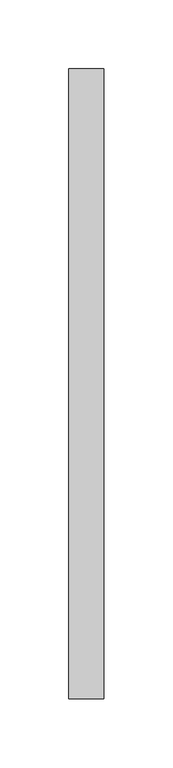
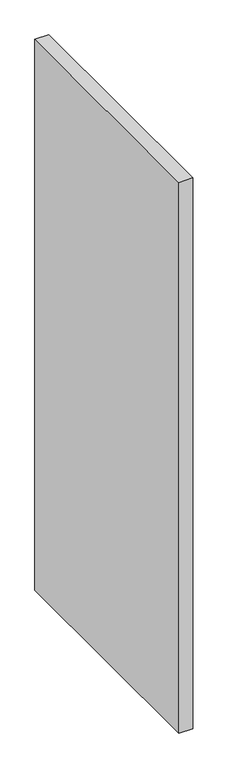
"""IFC4 building model written with IfcOpenShell, lengths in millimetres: proxy geometry."""

import ifcopenshell
import ifcopenshell.guid

model = None  # the IFC model being written
_history = None  # IfcOwnerHistory: only IFC2X3 demands one
_inside = {}  # id of a spatial element -> (the spatial element, [elements in it])
_under = {}  # id of a project, library or spatial element -> (it, [spatial elements below it])
_declared = {}  # id of a project -> (the project, [libraries it declares])
_typed = {}  # id of a type object -> (the type object, [elements of that type])
_made_of = {}  # id of a material, layer set ... -> (it, [elements and type objects made of it])


def new_model(schema):
    """Start an empty IFC model of exactly this schema.

    Asked for "IFC4X3", IfcOpenShell would pick the latest addendum, in which some entities
    have other attributes; the version numbers below select the first issue.
    IFC2X3 requires an IfcOwnerHistory on every rooted entity: one is made here for all.
    """
    global model, _history
    if schema == "IFC4X3":
        model = ifcopenshell.file(schema_version=(4, 3, 0, 0))
    else:
        model = ifcopenshell.file(schema=schema)
    _inside.clear()
    _under.clear()
    _declared.clear()
    _typed.clear()
    _made_of.clear()
    _history = None
    if model.schema == "IFC2X3":
        org = make("IfcOrganization", Name="unknown")
        user = make(
            "IfcPersonAndOrganization",
            ThePerson=make("IfcPerson", FamilyName="unknown"),
            TheOrganization=org,
        )
        app = make(
            "IfcApplication",
            ApplicationDeveloper=org,
            Version="unknown",
            ApplicationFullName="unknown",
            ApplicationIdentifier="unknown",
        )
        _history = make(
            "IfcOwnerHistory",
            OwningUser=user,
            OwningApplication=app,
            ChangeAction="ADDED",
            CreationDate=0,
        )
    return model


def make(cls, **values):
    """One entity of the class cls with the attributes given. An attribute that is None is left unset."""
    return model.create_entity(
        cls, **{name: value for name, value in values.items() if value is not None}
    )


def rooted(cls, **values):
    """An entity with a GlobalId (a new one), such as an element, a storey or a relation."""
    return make(cls, GlobalId=ifcopenshell.guid.new(), OwnerHistory=_history, **values)


def si_unit(unit_type, name, prefix=None):
    """IfcSIUnit, for example si_unit("LENGTHUNIT", "METRE", prefix="MILLI")."""
    return make("IfcSIUnit", UnitType=unit_type, Prefix=prefix, Name=name)


def assignment(units):
    """IfcUnitAssignment: the units of a project."""
    return None if units is None else make("IfcUnitAssignment", Units=units)


def point(xyz):
    """IfcCartesianPoint."""
    return None if xyz is None else make("IfcCartesianPoint", Coordinates=xyz)


def direction(xyz):
    """IfcDirection."""
    return None if xyz is None else make("IfcDirection", DirectionRatios=xyz)


def frame(location, z_axis=None, x_axis=None):
    """IfcAxis2Placement3D, a coordinate frame: its origin and axes. An axis left out is left unset."""
    return make(
        "IfcAxis2Placement3D",
        Location=point(location),
        Axis=direction(z_axis),
        RefDirection=direction(x_axis),
    )


def origin():
    """The frame at (0, 0, 0) with its axes left unset."""
    return frame((0.0, 0.0, 0.0))


def place(relative_to, where):
    """IfcLocalPlacement: puts the frame where relative to a parent placement (None: the world)."""
    return make(
        "IfcLocalPlacement", PlacementRelTo=relative_to, RelativePlacement=where
    )


def context(
    kind, dimensions, precision=None, world=None, true_north=None, identifier=None
):
    """IfcGeometricRepresentationContext, for example the 3D "Model" context."""
    return make(
        "IfcGeometricRepresentationContext",
        ContextIdentifier=identifier,
        ContextType=kind,
        CoordinateSpaceDimension=dimensions,
        Precision=precision,
        WorldCoordinateSystem=world,
        TrueNorth=true_north,
    )


def project(units=None, contexts=None):
    """IfcProject with its units and contexts."""
    return rooted(
        "IfcProject",
        Name="project",
        RepresentationContexts=contexts,
        UnitsInContext=assignment(units),
    )


def spatial(cls, under=None, at=None, **own):
    """A site, building, storey or space (cls), placed at a placement, below another one or the project."""
    s = rooted(cls, ObjectPlacement=at, **own)
    if under is not None:
        _under.setdefault(under.id(), (under, []))[1].append(s)
    return s


def polyline(points):
    """IfcPolyline through the points."""
    return make("IfcPolyline", Points=[point(p) for p in points])


def outline(outer, holes=None, kind="AREA"):
    """IfcArbitraryClosedProfileDef: a profile drawn as a closed curve; with holes, ...WithVoids."""
    if holes is None:
        return make("IfcArbitraryClosedProfileDef", ProfileType=kind, OuterCurve=outer)
    return make(
        "IfcArbitraryProfileDefWithVoids",
        ProfileType=kind,
        OuterCurve=outer,
        InnerCurves=holes,
    )


def extrude(swept, where, along, depth):
    """IfcExtrudedAreaSolid: the profile swept, set in the frame where, extruded along a direction by depth."""
    return make(
        "IfcExtrudedAreaSolid",
        SweptArea=swept,
        Position=where,
        ExtrudedDirection=direction(along),
        Depth=depth,
    )


def shape(context_of_items, identifier, shape_type, items):
    """IfcShapeRepresentation: the items that make up one representation, for example the "Body"."""
    return make(
        "IfcShapeRepresentation",
        ContextOfItems=context_of_items,
        RepresentationIdentifier=identifier,
        RepresentationType=shape_type,
        Items=items,
    )


def source(mapping_origin, context_of_items, identifier, shape_type, items):
    """IfcRepresentationMap: a shape defined once, which mapped items show again and again."""
    return make(
        "IfcRepresentationMap",
        MappingOrigin=mapping_origin,
        MappedRepresentation=shape(context_of_items, identifier, shape_type, items),
    )


def transform(
    local_origin,
    x_axis=None,
    y_axis=None,
    z_axis=None,
    scale=None,
    scale2=None,
    scale3=None,
    uniform=True,
):
    """IfcCartesianTransformationOperator3D, or its non-uniform kind. x_axis, y_axis, z_axis: its Axis1, 2, 3."""
    if uniform:
        return make(
            "IfcCartesianTransformationOperator3D",
            Axis1=direction(x_axis),
            Axis2=direction(y_axis),
            LocalOrigin=point(local_origin),
            Scale=scale,
            Axis3=direction(z_axis),
        )
    return make(
        "IfcCartesianTransformationOperator3DnonUniform",
        Axis1=direction(x_axis),
        Axis2=direction(y_axis),
        LocalOrigin=point(local_origin),
        Scale=scale,
        Axis3=direction(z_axis),
        Scale2=scale2,
        Scale3=scale3,
    )


def mapped(mapping_source, mapping_target):
    """IfcMappedItem: shows the shape of a source again, moved by a transform."""
    return make(
        "IfcMappedItem", MappingSource=mapping_source, MappingTarget=mapping_target
    )


def made_of(thing, what):
    """Note that an element or type object is made of a material, layer set ...; save() writes the relation."""
    if what is not None:
        _made_of.setdefault(what.id(), (what, []))[1].append(thing)
    return thing


def element(
    cls,
    number,
    at=None,
    inside=None,
    cuts=None,
    type_object=None,
    material=None,
    context=None,
    identifier="Body",
    shape_type=None,
    held_by="IfcProductDefinitionShape",
    body=None,
    shapes=None,
    **own,
):
    """One element of the class cls, such as IfcWall. Its Tag is "e" and its number.

    at: its placement. inside: the storey or other place that contains it. cuts: it is an
    opening in that element (IfcRelVoidsElement). A single representation is given by context,
    identifier, shape_type and body (its items); several are given by shapes. held_by: the class
    of the entity that holds the representations. save() writes the other relations.
    """
    e = rooted(cls, Tag="e%d" % number, ObjectPlacement=at, **own)
    if body is not None:
        shapes = [shape(context, identifier, shape_type, body)]
    if shapes is not None:
        e.Representation = make(held_by, Representations=shapes)
    if inside is not None:
        _inside.setdefault(inside.id(), (inside, []))[1].append(e)
    if cuts is not None:
        rooted(
            "IfcRelVoidsElement", RelatingBuildingElement=cuts, RelatedOpeningElement=e
        )
    if type_object is not None:
        _typed.setdefault(type_object.id(), (type_object, []))[1].append(e)
    return made_of(e, material)


def aggregate(whole, parts):
    """IfcRelAggregates: a whole, such as a stair, and the parts it consists of."""
    return rooted("IfcRelAggregates", RelatingObject=whole, RelatedObjects=parts)


def save(model, path):
    """Write the relations noted so far, then the file.

    IfcRelAggregates (storeys below a building ...), IfcRelContainedInSpatialStructure (elements
    in a storey), IfcRelDefinesByType, IfcRelAssociatesMaterial and IfcRelDeclares: one each for
    every whole, place, type object, material and project.
    """
    for whole, parts in _under.values():
        aggregate(whole, parts)
    for where, things in _inside.values():
        rooted(
            "IfcRelContainedInSpatialStructure",
            RelatedElements=things,
            RelatingStructure=where,
        )
    for kind, things in _typed.values():
        rooted("IfcRelDefinesByType", RelatedObjects=things, RelatingType=kind)
    for what, things in _made_of.values():
        rooted("IfcRelAssociatesMaterial", RelatedObjects=things, RelatingMaterial=what)
    for by, libraries in _declared.values():
        rooted("IfcRelDeclares", RelatingContext=by, RelatedDefinitions=libraries)
    model.write(path)


def specialty_equipment_2d138f7b(model_context):
    return source(origin(), model_context, "Body", "SweptSolid", [
        extrude(outline(polyline([(12.7, -198.4375), (12.7, -655.6375), (-12.7, -655.6375), (-12.7, -198.4375), (12.7, -198.4375)])), frame((0.0, 0.0, 355.6), z_axis=(0.0, 0.0, 1.0), x_axis=(1.0, 0.0, 0.0)), (0.0, 0.0, 1.0), 1066.8),
    ])


if __name__ == "__main__":
    model = new_model("IFC4")
    model_context = context("Model", 3, world=origin())
    ifc_project = project(units=[si_unit("LENGTHUNIT", "METRE", prefix="MILLI")], contexts=[model_context])
    site = spatial("IfcSite", under=ifc_project)
    building = spatial("IfcBuilding", under=site)
    placement = place(None, origin())
    specialty_equipment_shape = specialty_equipment_2d138f7b(model_context)
    element("IfcBuildingElementProxy", 1, Name="Urinal Screen-3D w Urinal : 36\" O.C.", ObjectType="Urinal Screen-3D w Urinal : 36\" O.C.", at=placement, inside=building, context=model_context, shape_type="MappedRepresentation", body=[
        mapped(specialty_equipment_shape, transform((0.0, 0.0, 0.0), x_axis=(1.0, 0.0, 0.0), y_axis=(0.0, 1.0, 0.0), z_axis=(0.0, 0.0, 1.0))),
    ])
    save(model, "model.ifc")

# Revit data of these elements
# Type "Urinal Screen-3D w Urinal : 36\" O.C."
#   Assembly Code = "C1030100"
#   O.C. = 3' - 0"
#   Depth = 1' - 6"
#   Toilet Partition Material = Toilet Partition
#   Default Elevation = 0
# Element 1 (IfcBuildingElementProxy, "Urinal Screen-3D w Urinal : 36\" O.C.")
#   Materials on its faces: "Toilet Partition"
# Materials
#   "Toilet Partition": class "Unassigned", colour RGB 0 181 188, transparency 0
